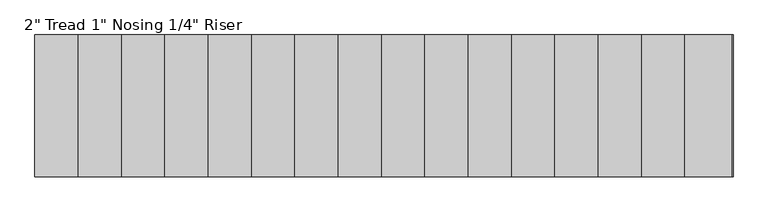
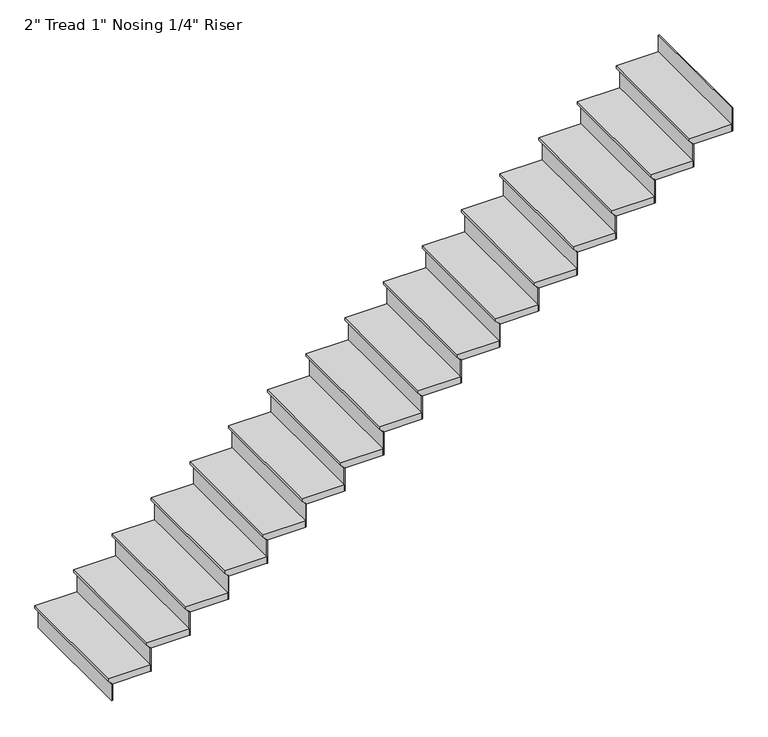
"""IFC4 building model written with IfcOpenShell, lengths in millimetres: stair flight geometry."""

from ifc_helpers import new_model, si_unit, frame, origin, place, context, project, spatial, polyline, outline, extrude, source, transform, mapped, element, save


def stair_flight_b20a5681(model_context):
    return source(origin(), model_context, "Body", "SweptSolid", [
        extrude(outline(polyline([(1887.4680756, 1038.4922402), (1887.4680756, 733.6922402), (1868.4180756, 733.6922402), (1843.0180756, 759.0922402), (1836.6680756, 759.0922402), (1836.6680756, 1038.4922402), (1887.4680756, 1038.4922402)])), frame((0.0, -11806.8919886, 0.0), z_axis=(0.0, 1.0, 0.0), x_axis=(0.0, 0.0, 1.0)), (0.0, 0.0, 1.0), 914.4),
        extrude(outline(polyline([(765.4422402, -11806.8919886), (759.0922402, -11806.8919886), (759.0922402, -10892.4919886), (765.4422402, -10892.4919886), (765.4422402, -11806.8919886)])), frame((0.0, 0.0, 1710.9974874), z_axis=(0.0, 0.0, 1.0), x_axis=(1.0, 0.0, 0.0)), (0.0, 0.0, 1.0), 125.6705882),
        extrude(outline(polyline([(1044.8422402, -11806.8919886), (1038.4922402, -11806.8919886), (1038.4922402, -10892.4919886), (1044.8422402, -10892.4919886), (1044.8422402, -11806.8919886)])), frame((0.0, 0.0, 1836.6680756), z_axis=(0.0, 0.0, 1.0), x_axis=(1.0, 0.0, 0.0)), (0.0, 0.0, 1.0), 176.4705882),
        extrude(outline(polyline([(2063.9386639, 1317.8922402), (2063.9386639, 1013.0922402), (2044.8886639, 1013.0922402), (2019.4886639, 1038.4922402), (2013.1386639, 1038.4922402), (2013.1386639, 1317.8922402), (2063.9386639, 1317.8922402)])), frame((0.0, -11806.8919886, 0.0), z_axis=(0.0, 1.0, 0.0), x_axis=(0.0, 0.0, 1.0)), (0.0, 0.0, 1.0), 914.4),
        extrude(outline(polyline([(1324.2422402, -11806.8919886), (1317.8922402, -11806.8919886), (1317.8922402, -10892.4919886), (1324.2422402, -10892.4919886), (1324.2422402, -11806.8919886)])), frame((0.0, 0.0, 2013.1386639), z_axis=(0.0, 0.0, 1.0), x_axis=(1.0, 0.0, 0.0)), (0.0, 0.0, 1.0), 176.4705882),
        extrude(outline(polyline([(2240.4092521, 1597.2922402), (2240.4092521, 1292.4922402), (2221.3592521, 1292.4922402), (2195.9592521, 1317.8922402), (2189.6092521, 1317.8922402), (2189.6092521, 1597.2922402), (2240.4092521, 1597.2922402)])), frame((0.0, -11806.8919886, 0.0), z_axis=(0.0, 1.0, 0.0), x_axis=(0.0, 0.0, 1.0)), (0.0, 0.0, 1.0), 914.4),
        extrude(outline(polyline([(1603.6422402, -11806.8919886), (1597.2922402, -11806.8919886), (1597.2922402, -10892.4919886), (1603.6422402, -10892.4919886), (1603.6422402, -11806.8919886)])), frame((0.0, 0.0, 2189.6092521), z_axis=(0.0, 0.0, 1.0), x_axis=(1.0, 0.0, 0.0)), (0.0, 0.0, 1.0), 176.4705882),
        extrude(outline(polyline([(2416.8798403, 1876.6922402), (2416.8798403, 1571.8922402), (2397.8298403, 1571.8922402), (2372.4298403, 1597.2922402), (2366.0798403, 1597.2922402), (2366.0798403, 1876.6922402), (2416.8798403, 1876.6922402)])), frame((0.0, -11806.8919886, 0.0), z_axis=(0.0, 1.0, 0.0), x_axis=(0.0, 0.0, 1.0)), (0.0, 0.0, 1.0), 914.4),
        extrude(outline(polyline([(1883.0422402, -11806.8919886), (1876.6922402, -11806.8919886), (1876.6922402, -10892.4919886), (1883.0422402, -10892.4919886), (1883.0422402, -11806.8919886)])), frame((0.0, 0.0, 2366.0798403), z_axis=(0.0, 0.0, 1.0), x_axis=(1.0, 0.0, 0.0)), (0.0, 0.0, 1.0), 176.4705882),
        extrude(outline(polyline([(2593.3504286, 2156.0922402), (2593.3504286, 1851.2922402), (2574.3004286, 1851.2922402), (2548.9004286, 1876.6922402), (2542.5504286, 1876.6922402), (2542.5504286, 2156.0922402), (2593.3504286, 2156.0922402)])), frame((0.0, -11806.8919886, 0.0), z_axis=(0.0, 1.0, 0.0), x_axis=(0.0, 0.0, 1.0)), (0.0, 0.0, 1.0), 914.4),
        extrude(outline(polyline([(2162.4422402, -11806.8919886), (2156.0922402, -11806.8919886), (2156.0922402, -10892.4919886), (2162.4422402, -10892.4919886), (2162.4422402, -11806.8919886)])), frame((0.0, 0.0, 2542.5504286), z_axis=(0.0, 0.0, 1.0), x_axis=(1.0, 0.0, 0.0)), (0.0, 0.0, 1.0), 176.4705882),
        extrude(outline(polyline([(2769.8210168, 2435.4922402), (2769.8210168, 2130.6922402), (2750.7710168, 2130.6922402), (2725.3710168, 2156.0922402), (2719.0210168, 2156.0922402), (2719.0210168, 2435.4922402), (2769.8210168, 2435.4922402)])), frame((0.0, -11806.8919886, 0.0), z_axis=(0.0, 1.0, 0.0), x_axis=(0.0, 0.0, 1.0)), (0.0, 0.0, 1.0), 914.4),
        extrude(outline(polyline([(2441.8422402, -11806.8919886), (2435.4922402, -11806.8919886), (2435.4922402, -10892.4919886), (2441.8422402, -10892.4919886), (2441.8422402, -11806.8919886)])), frame((0.0, 0.0, 2719.0210168), z_axis=(0.0, 0.0, 1.0), x_axis=(1.0, 0.0, 0.0)), (0.0, 0.0, 1.0), 176.4705882),
        extrude(outline(polyline([(2946.2916051, 2714.8922402), (2946.2916051, 2410.0922402), (2927.2416051, 2410.0922402), (2901.8416051, 2435.4922402), (2895.4916051, 2435.4922402), (2895.4916051, 2714.8922402), (2946.2916051, 2714.8922402)])), frame((0.0, -11806.8919886, 0.0), z_axis=(0.0, 1.0, 0.0), x_axis=(0.0, 0.0, 1.0)), (0.0, 0.0, 1.0), 914.4),
        extrude(outline(polyline([(2721.2422402, -11806.8919886), (2714.8922402, -11806.8919886), (2714.8922402, -10892.4919886), (2721.2422402, -10892.4919886), (2721.2422402, -11806.8919886)])), frame((0.0, 0.0, 2895.4916051), z_axis=(0.0, 0.0, 1.0), x_axis=(1.0, 0.0, 0.0)), (0.0, 0.0, 1.0), 176.4705882),
        extrude(outline(polyline([(3122.7621933, 2994.2922402), (3122.7621933, 2689.4922402), (3103.7121933, 2689.4922402), (3078.3121933, 2714.8922402), (3071.9621933, 2714.8922402), (3071.9621933, 2994.2922402), (3122.7621933, 2994.2922402)])), frame((0.0, -11806.8919886, 0.0), z_axis=(0.0, 1.0, 0.0), x_axis=(0.0, 0.0, 1.0)), (0.0, 0.0, 1.0), 914.4),
        extrude(outline(polyline([(3000.6422402, -11806.8919886), (2994.2922402, -11806.8919886), (2994.2922402, -10892.4919886), (3000.6422402, -10892.4919886), (3000.6422402, -11806.8919886)])), frame((0.0, 0.0, 3071.9621933), z_axis=(0.0, 0.0, 1.0), x_axis=(1.0, 0.0, 0.0)), (0.0, 0.0, 1.0), 176.4705882),
        extrude(outline(polyline([(3299.2327815, 3273.6922402), (3299.2327815, 2968.8922402), (3280.1827815, 2968.8922402), (3254.7827815, 2994.2922402), (3248.4327815, 2994.2922402), (3248.4327815, 3273.6922402), (3299.2327815, 3273.6922402)])), frame((0.0, -11806.8919886, 0.0), z_axis=(0.0, 1.0, 0.0), x_axis=(0.0, 0.0, 1.0)), (0.0, 0.0, 1.0), 914.4),
        extrude(outline(polyline([(3280.0422402, -11806.8919886), (3273.6922402, -11806.8919886), (3273.6922402, -10892.4919886), (3280.0422402, -10892.4919886), (3280.0422402, -11806.8919886)])), frame((0.0, 0.0, 3248.4327815), z_axis=(0.0, 0.0, 1.0), x_axis=(1.0, 0.0, 0.0)), (0.0, 0.0, 1.0), 176.4705882),
        extrude(outline(polyline([(3475.7033698, 3553.0922402), (3475.7033698, 3248.2922402), (3456.6533698, 3248.2922402), (3431.2533698, 3273.6922402), (3424.9033698, 3273.6922402), (3424.9033698, 3553.0922402), (3475.7033698, 3553.0922402)])), frame((0.0, -11806.8919886, 0.0), z_axis=(0.0, 1.0, 0.0), x_axis=(0.0, 0.0, 1.0)), (0.0, 0.0, 1.0), 914.4),
        extrude(outline(polyline([(3559.4422402, -11806.8919886), (3553.0922402, -11806.8919886), (3553.0922402, -10892.4919886), (3559.4422402, -10892.4919886), (3559.4422402, -11806.8919886)])), frame((0.0, 0.0, 3424.9033698), z_axis=(0.0, 0.0, 1.0), x_axis=(1.0, 0.0, 0.0)), (0.0, 0.0, 1.0), 176.4705882),
        extrude(outline(polyline([(3652.173958, 3832.4922402), (3652.173958, 3527.6922402), (3633.123958, 3527.6922402), (3607.723958, 3553.0922402), (3601.373958, 3553.0922402), (3601.373958, 3832.4922402), (3652.173958, 3832.4922402)])), frame((0.0, -11806.8919886, 0.0), z_axis=(0.0, 1.0, 0.0), x_axis=(0.0, 0.0, 1.0)), (0.0, 0.0, 1.0), 914.4),
        extrude(outline(polyline([(3838.8422402, -11806.8919886), (3832.4922402, -11806.8919886), (3832.4922402, -10892.4919886), (3838.8422402, -10892.4919886), (3838.8422402, -11806.8919886)])), frame((0.0, 0.0, 3601.373958), z_axis=(0.0, 0.0, 1.0), x_axis=(1.0, 0.0, 0.0)), (0.0, 0.0, 1.0), 176.4705882),
        extrude(outline(polyline([(3828.6445462, 4111.8922402), (3828.6445462, 3807.0922402), (3809.5945462, 3807.0922402), (3784.1945462, 3832.4922402), (3777.8445462, 3832.4922402), (3777.8445462, 4111.8922402), (3828.6445462, 4111.8922402)])), frame((0.0, -11806.8919886, 0.0), z_axis=(0.0, 1.0, 0.0), x_axis=(0.0, 0.0, 1.0)), (0.0, 0.0, 1.0), 914.4),
        extrude(outline(polyline([(4118.2422402, -11806.8919886), (4111.8922402, -11806.8919886), (4111.8922402, -10892.4919886), (4118.2422402, -10892.4919886), (4118.2422402, -11806.8919886)])), frame((0.0, 0.0, 3777.8445462), z_axis=(0.0, 0.0, 1.0), x_axis=(1.0, 0.0, 0.0)), (0.0, 0.0, 1.0), 176.4705882),
        extrude(outline(polyline([(4005.1151345, 4391.2922402), (4005.1151345, 4086.4922402), (3986.0651345, 4086.4922402), (3960.6651345, 4111.8922402), (3954.3151345, 4111.8922402), (3954.3151345, 4391.2922402), (4005.1151345, 4391.2922402)])), frame((0.0, -11806.8919886, 0.0), z_axis=(0.0, 1.0, 0.0), x_axis=(0.0, 0.0, 1.0)), (0.0, 0.0, 1.0), 914.4),
        extrude(outline(polyline([(4397.6422402, -11806.8919886), (4391.2922402, -11806.8919886), (4391.2922402, -10892.4919886), (4397.6422402, -10892.4919886), (4397.6422402, -11806.8919886)])), frame((0.0, 0.0, 3954.3151345), z_axis=(0.0, 0.0, 1.0), x_axis=(1.0, 0.0, 0.0)), (0.0, 0.0, 1.0), 176.4705882),
        extrude(outline(polyline([(4181.5857227, 4670.6922402), (4181.5857227, 4365.8922402), (4162.5357227, 4365.8922402), (4137.1357227, 4391.2922402), (4130.7857227, 4391.2922402), (4130.7857227, 4670.6922402), (4181.5857227, 4670.6922402)])), frame((0.0, -11806.8919886, 0.0), z_axis=(0.0, 1.0, 0.0), x_axis=(0.0, 0.0, 1.0)), (0.0, 0.0, 1.0), 914.4),
        extrude(outline(polyline([(4677.0422402, -11806.8919886), (4670.6922402, -11806.8919886), (4670.6922402, -10892.4919886), (4677.0422402, -10892.4919886), (4677.0422402, -11806.8919886)])), frame((0.0, 0.0, 4130.7857227), z_axis=(0.0, 0.0, 1.0), x_axis=(1.0, 0.0, 0.0)), (0.0, 0.0, 1.0), 176.4705882),
        extrude(outline(polyline([(4358.0563109, 4950.0922402), (4358.0563109, 4645.2922402), (4339.0063109, 4645.2922402), (4313.6063109, 4670.6922402), (4307.2563109, 4670.6922402), (4307.2563109, 4950.0922402), (4358.0563109, 4950.0922402)])), frame((0.0, -11806.8919886, 0.0), z_axis=(0.0, 1.0, 0.0), x_axis=(0.0, 0.0, 1.0)), (0.0, 0.0, 1.0), 914.4),
        extrude(outline(polyline([(4956.4422402, -11806.8919886), (4950.0922402, -11806.8919886), (4950.0922402, -10892.4919886), (4956.4422402, -10892.4919886), (4956.4422402, -11806.8919886)])), frame((0.0, 0.0, 4307.2563109), z_axis=(0.0, 0.0, 1.0), x_axis=(1.0, 0.0, 0.0)), (0.0, 0.0, 1.0), 176.4705882),
        extrude(outline(polyline([(5235.8422402, -11806.8919886), (5229.4922402, -11806.8919886), (5229.4922402, -10892.4919886), (5235.8422402, -10892.4919886), (5235.8422402, -11806.8919886)])), frame((0.0, 0.0, 4483.7268992), z_axis=(0.0, 0.0, 1.0), x_axis=(1.0, 0.0, 0.0)), (0.0, 0.0, 1.0), 176.4705882),
        extrude(outline(polyline([(4534.5268992, 5229.4922402), (4534.5268992, 4924.6922402), (4515.4768992, 4924.6922402), (4490.0768992, 4950.0922402), (4483.7268992, 4950.0922402), (4483.7268992, 5229.4922402), (4534.5268992, 5229.4922402)])), frame((0.0, -11806.8919886, 0.0), z_axis=(0.0, 1.0, 0.0), x_axis=(0.0, 0.0, 1.0)), (0.0, 0.0, 1.0), 914.4),
    ])


if __name__ == "__main__":
    model = new_model("IFC4")
    model_context = context("Model", 3, world=origin())
    ifc_project = project(units=[si_unit("LENGTHUNIT", "METRE", prefix="MILLI")], contexts=[model_context])
    site = spatial("IfcSite", under=ifc_project)
    building = spatial("IfcBuilding", under=site)
    placement = place(None, origin())
    stair_flight_shape = stair_flight_b20a5681(model_context)
    element("IfcStairFlight", 1, ObjectType="2\" Tread 1\" Nosing 1/4\" Riser", at=placement, inside=building, context=model_context, shape_type="MappedRepresentation", body=[
        mapped(stair_flight_shape, transform((0.0, 0.0, 0.0), x_axis=(1.0, 0.0, 0.0), y_axis=(0.0, 1.0, 0.0), z_axis=(0.0, 0.0, 1.0))),
    ])
    save(model, "model.ifc")
